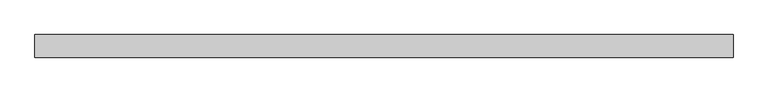
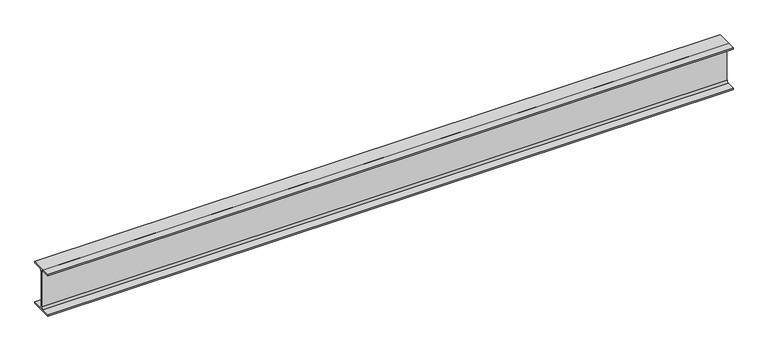
"""IFC4 building model written with IfcOpenShell, lengths in millimetres: beam geometry, 0912_Steel Framing_H-KSD3502 : H_SB_ASB_H-250x125x6x9."""

from ifc_helpers import new_model, si_unit, point, frame, frame_2d, origin, place, context, project, spatial, polyline, circle_curve, trimmed, segment, composite_curve, outline, extrude, source, transform, mapped, element, save


def beam_77ce1637(model_context):
    return source(origin(), model_context, "Body", "SweptSolid", [
        extrude(outline(composite_curve([segment(polyline([(62.5, -116.0), (62.5, -125.0), (-62.5, -125.0), (-62.5, -116.0), (-15.0, -116.0)]), True, "CONTINUOUS"), segment(trimmed(circle_curve(frame_2d((-15.0, -104.0)), 12.0), [point((-15.0, -116.0))], [point((-3.0, -104.0))], True, "CARTESIAN"), True, "CONTINUOUS"), segment(polyline([(-3.0, -104.0), (-3.0, 104.0)]), True, "CONTINUOUS"), segment(trimmed(circle_curve(frame_2d((-15.0, 104.0)), 12.0), [point((-3.0, 104.0))], [point((-15.0, 116.0))], True, "CARTESIAN"), True, "CONTINUOUS"), segment(polyline([(-15.0, 116.0), (-62.5, 116.0), (-62.5, 125.0), (62.5, 125.0), (62.5, 116.0), (15.0, 116.0)]), True, "CONTINUOUS"), segment(trimmed(circle_curve(frame_2d((15.0, 104.0)), 12.0), [point((15.0, 116.0))], [point((3.0, 104.0))], True, "CARTESIAN"), True, "CONTINUOUS"), segment(polyline([(3.0, 104.0), (3.0, -104.0)]), True, "CONTINUOUS"), segment(trimmed(circle_curve(frame_2d((15.0, -104.0)), 12.0), [point((3.0, -104.0))], [point((15.0, -116.0))], True, "CARTESIAN"), True, "CONTINUOUS"), segment(polyline([(15.0, -116.0), (62.5, -116.0)]), True, "CONTINUOUS")], self_intersect=False)), frame((-2029.8, 0.0, 0.0), z_axis=(1.0, 0.0, 0.0), x_axis=(0.0, 1.0, 0.0)), (0.0, 0.0, 1.0), 3859.8829189),
    ])


if __name__ == "__main__":
    model = new_model("IFC4")
    model_context = context("Model", 3, world=origin())
    ifc_project = project(units=[si_unit("LENGTHUNIT", "METRE", prefix="MILLI")], contexts=[model_context])
    site = spatial("IfcSite", under=ifc_project)
    building = spatial("IfcBuilding", under=site)
    placement = place(None, origin())
    beam_shape = beam_77ce1637(model_context)
    element("IfcBeam", 1, ObjectType="0912_Steel Framing_H-KSD3502 : H_SB_ASB_H-250x125x6x9", at=placement, inside=building, context=model_context, shape_type="MappedRepresentation", body=[
        mapped(beam_shape, transform((0.0, 0.0, 0.0), x_axis=(1.0, 0.0, 0.0), y_axis=(0.0, 1.0, 0.0), z_axis=(0.0, 0.0, 1.0))),
    ])
    save(model, "model.ifc")

# Revit data of these elements
# Type "0912_Steel Framing_H-KSD3502 : H_SB_ASB_H-250x125x6x9"
#   H_WM Code_1 = "S01AA003-00001 | Main Steel Structure Fabrication Work | Shelter/Building | Light Steel - Standard (30KG/M>Weight) | Material: (   )"
#   H_WM Code_2 = "S03AA029-00001 | Main Steel Structure Erection Work | Shelter/Building | Light Steel (30KG/M>Weight) | Material: (   )"
#   H_WM Code_3 = "S01AA010-00001 | Main Steel Structure Fabrication Work | Shelter/Building | Steel Painting/Coating | for Non-Fireproofed Steel Surface, Surface Preparation, Primer, Second & Final Coat | Material: (   )"
#   H_Q'ty Cal Type Tag = "SB-Q2"
#   Width = 12.5 cm
#   Web Thickness = 0.6 cm
#   Web Fillet = 1.2 cm
#   Warping Constant = 42539.8 cm⁶
#   W = 0
#   Torsional Moment of Inertia = 7.8102 cm⁴
#   Section Area = 37.66 cm²
#   Plastic Modulus weak axis = 73.1 cm³
#   Plastic Modulus strong axis = 366.0 cm³
#   Perimeter = 0.97 m²/m
#   Nominal Weight = 29.60 kgf/m
#   Moment of Inertia weak axis = 294.00 cm⁴
#   Moment of Inertia strong axis = 4050.00 cm⁴
#   Height = 25.0 cm
#   Flange Thickness = 0.9 cm
#   Elastic Modulus weak axis = 47.0 cm³
#   Elastic Modulus strong axis = 324.0 cm³
#   Centroid Vertical = 12.5 cm
#   Centroid Horizontal = 6.25 cm
#   Ix = 40500000
#   Length [instance default] = 1.5240 m
#   Zx = 366000
#   b = 0.1250 m
#   h = 0.2500 m
#   r = 0.0120 m
#   s = 0.0060 m
#   t = 0.0090 m
#   A = 0.003766 m²
#   Structural Material [instance default] = Steel, 45-345
#   Assembly Code = ""
# Element 1 (IfcBeam, "0912_Steel Framing_H-KSD3502 : H_SB_ASB_H-250x125x6x9")
#   Structural Material = none
# Materials
#   "Steel, 45-345": class "Metal", colour RGB 189 187 185, transparency 0, Description = "Steel 345 MPa", Cost = 0
